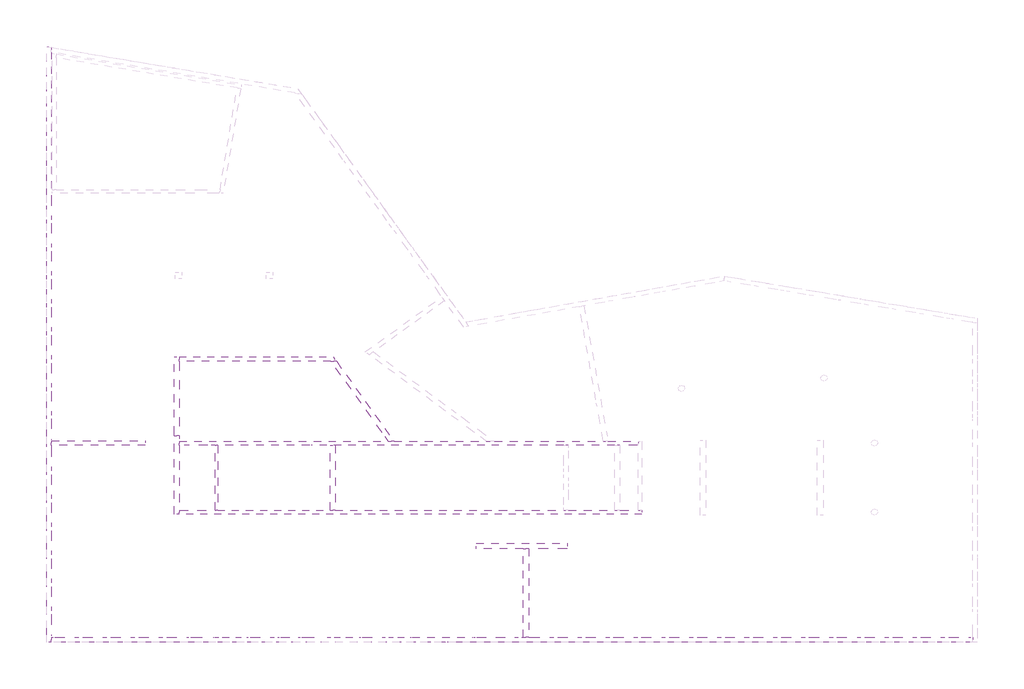
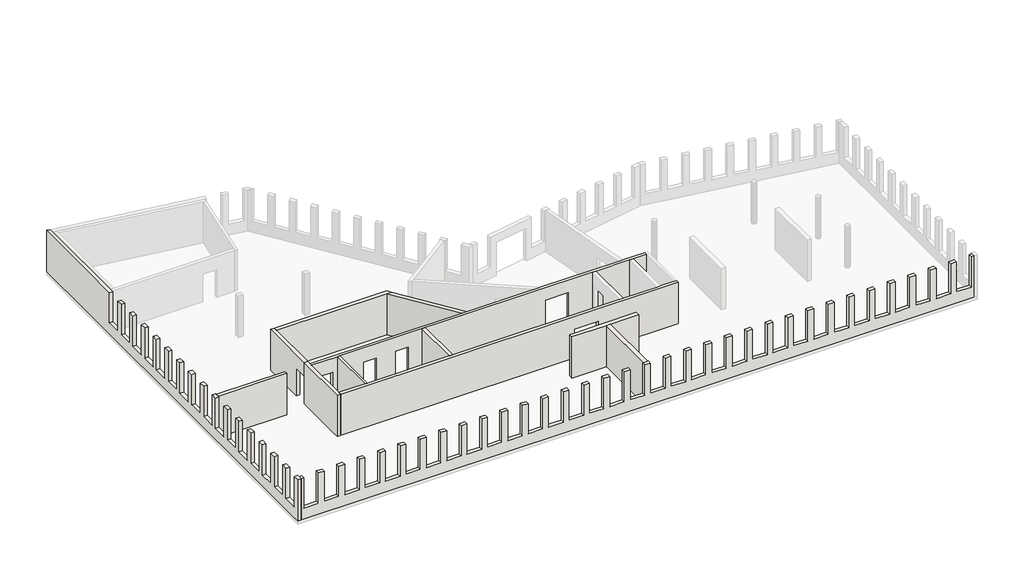
# One storey, part 1 of 2: 13 walls.
# Revit data of these elements (continued)
# Elements 7, 8 (IfcWall, "5dki STB-Wand Kern 22cm C30/37") (continued)
#   Base Constraint = 01_UG_OKRD_-0,15
#   Top Constraint = 00_EG_UKRD_3,06
#   Materials on its faces: "5d Beton - Stahlbeton"
# Element 10 (IfcWall, "5dki STB-Wand Kern 15cm C30/37")
#   Comments = ""
#   000_080_030_Geschoß = "00_EG"
#   Top Offset = 0.000 m
#   Base Offset = 0.000 m
#   wall height = 3.210 m
#   Phase Created = Neu
#   Base Constraint = 01_UG_OKRD_-0,15
#   Top Constraint = 00_EG_UKRD_3,06
#   Materials on its faces: "5d Beton - Stahlbeton"
# Element 11 (IfcWall, "5dki STB-Wand 25cm C30/37")
#   Comments = ""
#   000_080_030_Geschoß = "00_EG"
#   Top Offset = 0.000 m
#   Base Offset = 0.000 m
#   wall height = 3.210 m
#   Phase Created = Neu
#   Base Constraint = 01_UG_OKRD_-0,15
#   Top Constraint = 00_EG_UKRD_3,06
#   Materials on its faces: "5d Beton - Stahlbeton"
# Element 12 (IfcWall, "5dki STB-Wand 30cm C30/37")
#   Comments = ""
#   000_080_030_Geschoß = "00_EG"
#   Top Offset = 0.000 m
#   Base Offset = 0.000 m
#   wall height = 3.210 m
#   Phase Created = Neu
#   Base Constraint = 01_UG_OKRD_-0,15
#   Top Constraint = 00_EG_UKRD_3,06
#   Materials on its faces: "5d Beton - Stahlbeton"
# Element 13 (IfcWall, "5dki STB-Wand 30cm C30/37")
#   000_080_030_Geschoß = "00_EG"
#   Top Offset = 0.000 m
#   Base Offset = 0.000 m
#   wall height = 3.210 m
#   Phase Created = Neu
#   Base Constraint = 01_UG_OKRD_-0,15
#   Top Constraint = 00_EG_UKRD_3,06
#   Materials on its faces: "5d Beton - Stahlbeton"
# Materials
#   "5d Beton - Stahlbeton": class "5dki", colour RGB 200 200 200, transparency 0, Cost = 0
